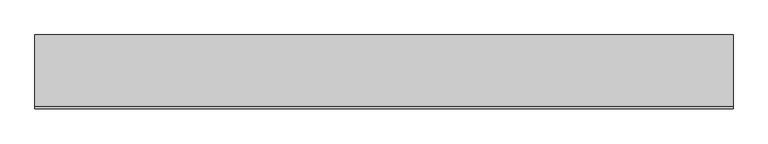
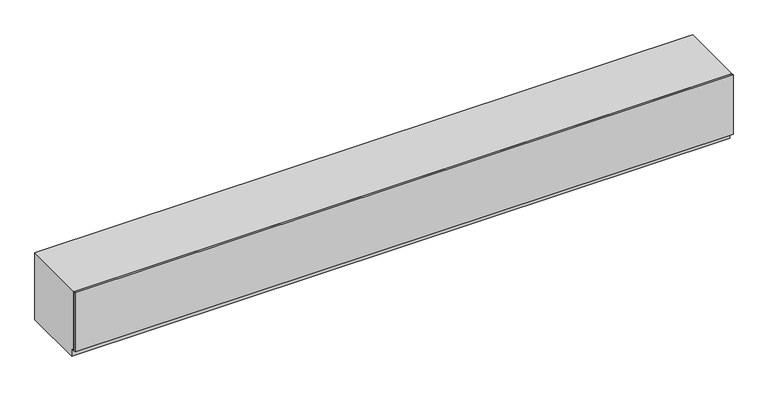
"""IFC4 building model written with IfcOpenShell, lengths in millimetres: furniture geometry, OD_CW_Base Cabinet : OD_CW_Base Cabinet."""

from ifc_helpers import new_model, si_unit, frame, origin, place, context, project, spatial, polyline, outline, extrude, source, transform, mapped, element, save


def furniture_2298d4ce(model_context):
    return source(origin(), model_context, "Body", "SweptSolid", [
        extrude(outline(polyline([(18.7377049, -228.6), (8167.5056128, -228.6), (8167.5056128, -254.0), (18.7377049, -254.0), (18.7377049, -228.6)])), frame((0.0, 0.0, 101.6), z_axis=(0.0, 0.0, 1.0), x_axis=(1.0, 0.0, 0.0)), (0.0, 0.0, 1.0), 774.7),
        extrude(outline(polyline([(-228.6, 876.3), (609.6, 876.3), (609.6, 0.0), (-177.8, 0.0), (-177.8, 101.6), (-228.6, 101.6), (-228.6, 876.3)])), frame((18.7377049, 0.0, 0.0), z_axis=(1.0, 0.0, 0.0), x_axis=(0.0, 1.0, 0.0)), (0.0, 0.0, 1.0), 8148.7679079),
    ])


if __name__ == "__main__":
    model = new_model("IFC4")
    model_context = context("Model", 3, world=origin())
    ifc_project = project(units=[si_unit("LENGTHUNIT", "METRE", prefix="MILLI")], contexts=[model_context])
    site = spatial("IfcSite", under=ifc_project)
    building = spatial("IfcBuilding", under=site)
    placement = place(None, origin())
    furniture_shape = furniture_2298d4ce(model_context)
    element("IfcFurniture", 1, ObjectType="OD_CW_Base Cabinet : OD_CW_Base Cabinet", at=placement, inside=building, context=model_context, shape_type="MappedRepresentation", body=[
        mapped(furniture_shape, transform((0.0, 0.0, 0.0), x_axis=(1.0, 0.0, 0.0), y_axis=(0.0, 1.0, 0.0), z_axis=(0.0, 0.0, 1.0))),
    ])
    save(model, "model.ifc")

# Revit data of these elements
# Type "OD_CW_Base Cabinet : OD_CW_Base Cabinet"
#   OD_CW_Width [instance default] = 2' - 10"
#   OD_CW_Length [instance default] = 8' - 0"
#   OD_CW_Height [instance default] = 2' - 3"
#   Depth = 2' - 0"
#   Height = 3' - 0"
#   Width = 4' - 0"
#   OD_CW_Material_Front Panel [instance default] = none
#   OD_CW_Material_Body [instance default] = none
# Element 1 (IfcFurniture, "OD_CW_Base Cabinet : OD_CW_Base Cabinet")
#   OD_CW_Length = 26' - 8.81763"
#   OD_CW_Height = 2' - 10 1/2"
#   OD_CW_Material_Front Panel = WOOD-OAKFIRE
#   OD_CW_Material_Body = WOOD-OAKFIRE
#   Materials on its faces: "WOOD-OAKFIRE"
# Materials
#   "WOOD-OAKFIRE": class "Wood", colour RGB 198 202 183, transparency 0, Description = "Generic wood", Cost = 0
